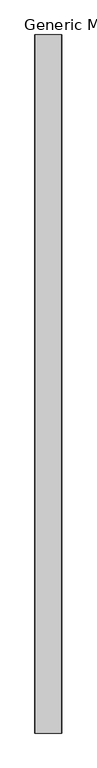
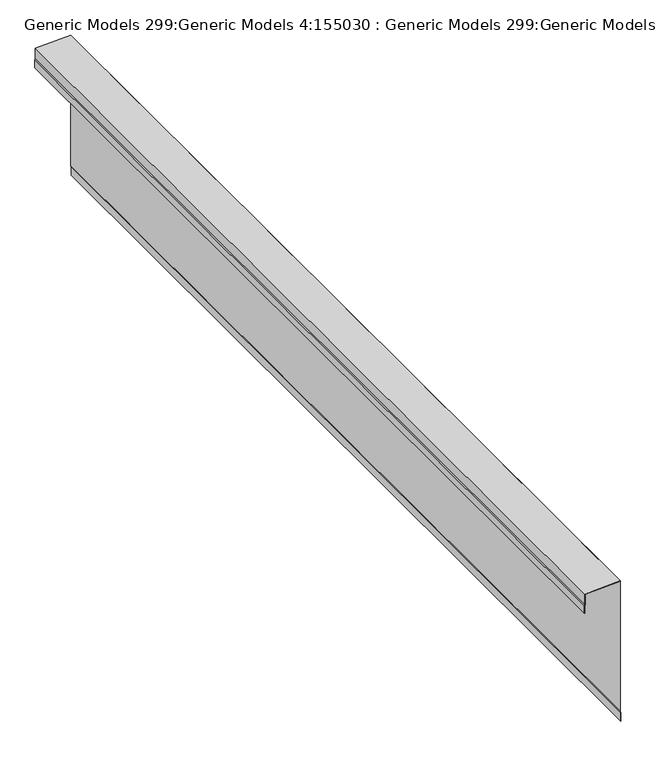
"""IFC4 building model written with IfcOpenShell, lengths in millimetres: proxy geometry, Generic Models 299:Generic Models 4:155030 : Generic Models 299:Generic Models 4:155030."""

from ifc_helpers import new_model, si_unit, frame, origin, place, context, project, spatial, polyline, outline, extrude, source, transform, mapped, element, save


def generic_models_299_generic_models_4_155030_generic_models_f908ff86(model_context):
    return source(origin(), model_context, "Body", "SweptSolid", [
        extrude(outline(polyline([(801.569527, 6646.129274), (840.8201708, 6646.129274), (847.9521113, 6648.725088), (905.65918, 6648.725088), (913.2389413, 6830.6393587), (200.552059, 6830.6393587), (190.7778748, 6834.1968708), (146.6009052, 6834.1968708), (146.6009052, 6835.0822598), (190.6660583, 6835.0822598), (200.6920186, 6831.4331087), (914.0664529, 6831.4331087), (906.4205458, 6647.931338), (848.0920709, 6647.931338), (840.9601303, 6645.335524), (801.569527, 6645.335524), (801.569527, 6646.129274)])), frame((0.0, 7041.2025207, 0.0), z_axis=(0.0, 1.0, 0.0), x_axis=(0.0, 0.0, 1.0)), (0.0, 0.0, 1.0), 4927.6),
    ])


if __name__ == "__main__":
    model = new_model("IFC4")
    model_context = context("Model", 3, world=origin())
    ifc_project = project(units=[si_unit("LENGTHUNIT", "METRE", prefix="MILLI")], contexts=[model_context])
    site = spatial("IfcSite", under=ifc_project)
    building = spatial("IfcBuilding", under=site)
    placement = place(None, origin())
    generic_models_299_generic_models_4_155030_generic_models_shape = generic_models_299_generic_models_4_155030_generic_models_f908ff86(model_context)
    element("IfcBuildingElementProxy", 1, Name="Generic Models 299:Generic Models 4:155030 : Generic Models 299:Generic Models 4:155030", ObjectType="Generic Models 299:Generic Models 4:155030 : Generic Models 299:Generic Models 4:155030", at=placement, inside=building, context=model_context, shape_type="MappedRepresentation", body=[
        mapped(generic_models_299_generic_models_4_155030_generic_models_shape, transform((0.0, 0.0, 0.0), x_axis=(1.0, 0.0, 0.0), y_axis=(0.0, 1.0, 0.0), z_axis=(0.0, 0.0, 1.0))),
    ])
    save(model, "model.ifc")

# Revit data of these elements
# Type "Generic Models 299:Generic Models 4:155030 : Generic Models 299:Generic Models 4:155030"
#   NameOverride = "Generic Models 299:Generic Models 4:155030"
#   ObjectTypeOverride = "Generic Models 299:Generic Models 4"
#   Reference = "Generic Models 4"
#   Category = "Generic Models"
#   Tag = "155030"
# Element 1 (IfcBuildingElementProxy, "Generic Models 299:Generic Models 4:155030 : Generic Models 299:Generic Models 4:155030")
#   Materials on its faces: "_(2) LAYERS NO. 30 ASTM D226 ASPHALT SATURATED ORGANIC FELT 997"
# Materials
#   "_(2) LAYERS NO. 30 ASTM D226 ASPHALT SATURATED ORGANIC FELT 997": class "Unassigned", colour RGB 67 154 161, transparency 0
